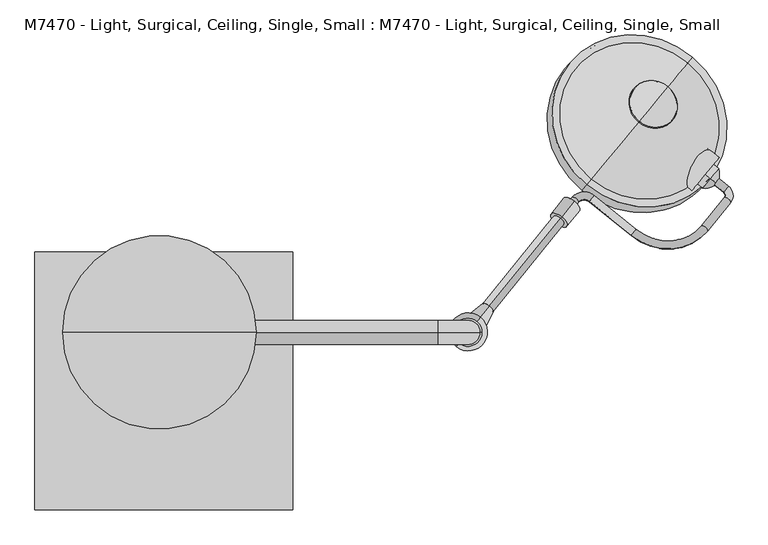
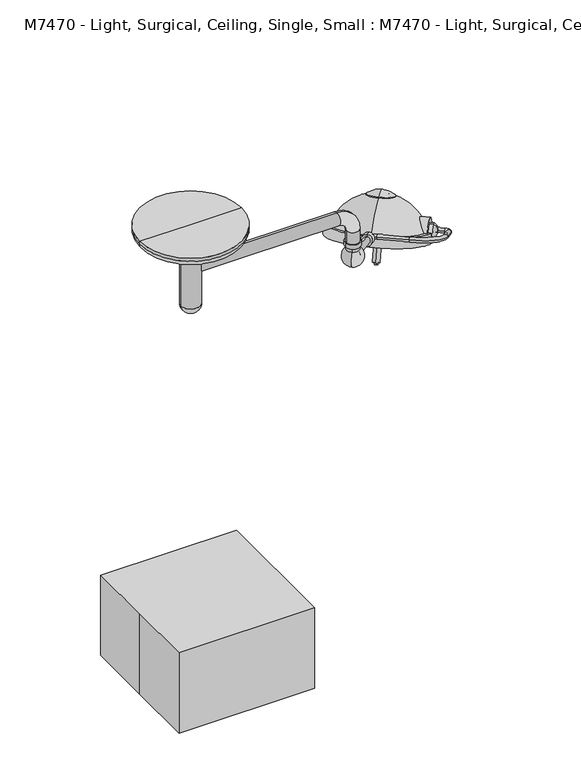
"""IFC4 building model written with IfcOpenShell, lengths in millimetres: proxy geometry, M7470 - Light, Surgical, Ceiling, Single, Small : M7470 - Light, Surgical, Ceiling, Single, Small."""

from ifc_helpers import new_model, si_unit, point, frame, frame_2d, origin, origin_with_axes, origin_2d, place, context, project, spatial, polyline, circle_curve, ellipse_curve, trimmed, segment, composite_curve, outline, extrude, source, transform, mapped, element, save
from ifc_brep_helpers import plane_surface, cylinder_surface, revolved_surface, advanced_brep


def m7470_light_surgical_ceiling_single_small_m7470_light_7ae27e33(model_context):
    return source(origin(), model_context, "Body", "SolidModel", [
        advanced_brep(
        [(1740.835031, 642.2802758, 1801.3604265), (1726.2322463, 624.2473385, 1811.6915373), (1762.8864892, 594.5653179, 1811.6915373), (1777.4892739, 612.5982552, 1801.3604265), (1765.4548505, 577.5564802, 1816.8570926), (1785.194358, 561.5717423, 1816.8570926), (1692.9754347, 488.0518556, 1868.1344952), (1712.7149421, 472.0671177, 1868.1344952), (1486.9216817, 475.7626592, 1930.1211596), (1472.318897, 457.7297218, 1940.4522704), (1355.271585, 582.3708055, 1930.1211596), (1340.6688003, 564.3378681, 1940.4522704), (1286.5870007, 578.2744067, 1950.7833811), (1306.3265081, 562.2896687, 1950.7833811), (1251.0372497, 494.0131207, 1989.8991704), (1231.2977423, 509.9978587, 1989.8991704)],
        [
            (0, 1, circle_curve(frame((1733.5336387, 633.2638072, 1806.5259819), z_axis=(-0.7771459614569792, 0.6293203910498273, 0.0), x_axis=(-0.5749127846454345, -0.7099581630143155, 0.40673664307580054)), 12.7)),
            (1, 0, circle_curve(frame((1733.5336387, 633.2638072, 1806.5259819), z_axis=(-0.7771459614569792, 0.6293203910498273, 0.0), x_axis=(-0.5749127846454345, -0.7099581630143155, 0.40673664307580054)), 12.7)),
            (1, 2),
            (2, 3, circle_curve(frame((1770.1878816, 603.5817865, 1806.5259819), z_axis=(-0.7771459614569792, 0.6293203910498273, 0.0), x_axis=(-0.5749127846454345, -0.7099581630143155, 0.40673664307580054)), 12.7)),
            (3, 0),
            (3, 2, circle_curve(frame((1770.1878816, 603.5817865, 1806.5259819), z_axis=(-0.7771459614569792, 0.6293203910498273, 0.0), x_axis=(-0.5749127846454345, -0.7099581630143155, 0.40673664307580054)), 12.7)),
            (4, 5, circle_curve(frame((1775.3246043, 569.5641113, 1816.8570926), z_axis=(0.574912784645419, 0.709958163014328, -0.4067366430758005), x_axis=(-0.7771459614569908, 0.6293203910498131, 0.0)), 12.7)),
            (5, 3, circle_curve(frame((1755.5850968, 585.5488492, 1816.8570926), z_axis=(0.2559676632747577, 0.31609373954292624, 0.9135454576426008), x_axis=(0.5749127846454357, 0.7099581630143145, -0.4067366430758004)), 38.1)),
            (2, 4, circle_curve(frame((1755.5850968, 585.5488492, 1816.8570926), z_axis=(-0.2559676632747577, -0.31609373954292624, -0.9135454576426008), x_axis=(0.5749127846454357, 0.7099581630143145, -0.4067366430758004)), 12.7)),
            (5, 4, circle_curve(frame((1775.3246043, 569.5641113, 1816.8570926), z_axis=(0.5749127846454273, 0.7099581630143212, -0.4067366430758005), x_axis=(-0.7771459614569847, 0.6293203910498207, 0.0)), 12.7)),
            (4, 6),
            (6, 7, circle_curve(frame((1702.8451884, 480.0594867, 1868.1344952), z_axis=(0.5749127846454346, 0.7099581630143152, -0.40673664307580043), x_axis=(-0.777145961456979, 0.6293203910498273, 0.0)), 12.7)),
            (7, 5),
            (7, 6, circle_curve(frame((1702.8451884, 480.0594867, 1868.1344952), z_axis=(0.5749127846454346, 0.7099581630143152, -0.40673664307580043), x_axis=(-0.777145961456979, 0.6293203910498273, 0.0)), 12.7)),
            (8, 9, circle_curve(frame((1479.6202894, 466.7461905, 1935.286715), z_axis=(0.7771459614569775, -0.6293203910498295, 0.0), x_axis=(0.5749127846454369, 0.7099581630143138, -0.4067366430758004)), 12.7)),
            (9, 7, circle_curve(frame((1574.5383901, 583.9602832, 1868.1344952), z_axis=(0.2559676632747577, 0.31609373954292624, 0.9135454576426008), x_axis=(0.7771459614569818, -0.6293203910498242, 0.0)), 177.8)),
            (6, 8, circle_curve(frame((1574.5383901, 583.9602832, 1868.1344952), z_axis=(-0.2559676632747577, -0.31609373954292624, -0.9135454576426008), x_axis=(0.7771459614569818, -0.6293203910498242, 0.0)), 152.4)),
            (9, 8, circle_curve(frame((1479.6202894, 466.7461905, 1935.286715), z_axis=(0.7771459614569785, -0.6293203910498282, 0.0), x_axis=(0.5749127846454356, 0.7099581630143149, -0.4067366430758004)), 12.7)),
            (8, 10),
            (10, 11, circle_curve(frame((1347.9701926, 573.3543368, 1935.286715), z_axis=(0.777145961456978, -0.6293203910498286, 0.0), x_axis=(0.574912784645436, 0.7099581630143144, -0.4067366430758003)), 12.7)),
            (11, 9),
            (11, 10, circle_curve(frame((1347.9701926, 573.3543368, 1935.286715), z_axis=(0.777145961456978, -0.6293203910498286, 0.0), x_axis=(0.574912784645436, 0.7099581630143144, -0.4067366430758003)), 12.7)),
            (12, 13, circle_curve(frame((1296.4567544, 570.2820377, 1950.7833811), z_axis=(0.5749127846454385, 0.7099581630143121, -0.40673664307580054), x_axis=(-0.7771459614569765, 0.629320391049831, 0.0)), 12.7)),
            (13, 11, circle_curve(frame((1326.0660155, 546.3049308, 1950.7833811), z_axis=(-0.2559676632747577, -0.31609373954292624, -0.9135454576426008), x_axis=(0.5749127846454407, 0.7099581630143105, -0.4067366430758004)), 25.4)),
            (10, 12, circle_curve(frame((1326.0660155, 546.3049308, 1950.7833811), z_axis=(0.2559676632747577, 0.31609373954292624, 0.9135454576426008), x_axis=(0.5749127846454407, 0.7099581630143105, -0.4067366430758004)), 50.8)),
            (13, 12, circle_curve(frame((1296.4567544, 570.2820377, 1950.7833811), z_axis=(0.5749127846454364, 0.7099581630143139, -0.40673664307580054), x_axis=(-0.777145961456978, 0.6293203910498291, 0.0)), 12.7)),
            (14, 15, circle_curve(frame((1241.167496, 502.0054897, 1989.8991704), z_axis=(-0.5749127846454374, -0.7099581630143132, 0.40673664307580004), x_axis=(-0.7771459614569771, 0.6293203910498298, 0.0)), 12.7)),
            (15, 14, circle_curve(frame((1241.167496, 502.0054897, 1989.8991704), z_axis=(-0.5749127846454374, -0.7099581630143132, 0.40673664307580004), x_axis=(-0.7771459614569771, 0.6293203910498298, 0.0)), 12.7)),
            (12, 15),
            (14, 13),
        ],
        [
            plane_surface(frame((1306.7585861, 106.2405083, 283.3710423), z_axis=(-0.7771459614569792, 0.6293203910498271, 0.0), x_axis=(0.2559676632747578, 0.3160937395429264, 0.9135454576426008))),
            cylinder_surface(frame((1733.5336387, 633.2638072, 1806.5259819), z_axis=(-0.7771459614569792, 0.6293203910498273, 0.0), x_axis=(-0.5749127846454345, -0.7099581630143155, 0.40673664307580054)), 12.7),
            revolved_surface(trimmed(ellipse_curve(frame((1770.1878816, 603.5817865, 1806.5259819), z_axis=(0.7771459614569786, -0.6293203910498283, 0.0), x_axis=(-0.5749127846454356, -0.7099581630143146, 0.40673664307580043)), 12.7, 12.7), [point((1777.4892739, 612.5982552, 1801.3604265))], [point((1762.8864892, 594.5653179, 1811.6915373))], True, "CARTESIAN"), (1328.8100443, 58.5255503, 293.7021531), (0.25596766327475773, 0.3160937395429263, 0.913545457642601)),
            revolved_surface(trimmed(ellipse_curve(frame((1770.1878816, 603.5817865, 1806.5259819), z_axis=(0.7771459614569786, -0.6293203910498283, 0.0), x_axis=(-0.5749127846454356, -0.7099581630143146, 0.40673664307580043)), 12.7, 12.7), [point((1762.8864892, 594.5653179, 1811.6915373))], [point((1777.4892739, 612.5982552, 1801.3604265))], True, "CARTESIAN"), (1328.8100443, 58.5255503, 293.7021531), (0.25596766327475773, 0.3160937395429263, 0.913545457642601)),
            cylinder_surface(frame((1775.3246043, 569.5641113, 1816.8570926), z_axis=(0.5749127846454346, 0.7099581630143152, -0.40673664307580043), x_axis=(-0.777145961456979, 0.6293203910498273, 0.0)), 12.7),
            revolved_surface(trimmed(ellipse_curve(frame((1702.8451884, 480.0594867, 1868.1344952), z_axis=(-0.5749127846454308, -0.7099581630143185, 0.4067366430758007), x_axis=(-0.777145961456982, 0.6293203910498238, 0.0)), 12.7, 12.7), [point((1712.7149421, 472.0671177, 1868.1344952))], [point((1692.9754347, 488.0518556, 1868.1344952))], True, "CARTESIAN"), (1147.7633376, 56.9369844, 344.9795556), (0.25596766327475773, 0.3160937395429263, 0.913545457642601)),
            revolved_surface(trimmed(ellipse_curve(frame((1702.8451884, 480.0594867, 1868.1344952), z_axis=(-0.5749127846454308, -0.7099581630143185, 0.4067366430758007), x_axis=(-0.777145961456982, 0.6293203910498238, 0.0)), 12.7, 12.7), [point((1692.9754347, 488.0518556, 1868.1344952))], [point((1712.7149421, 472.0671177, 1868.1344952))], True, "CARTESIAN"), (1147.7633376, 56.9369844, 344.9795556), (0.25596766327475773, 0.3160937395429263, 0.913545457642601)),
            cylinder_surface(frame((1479.6202894, 466.7461905, 1935.286715), z_axis=(0.7771459614569782, -0.6293203910498287, 0.0), x_axis=(0.574912784645436, 0.7099581630143144, -0.4067366430758003)), 12.7),
            revolved_surface(trimmed(ellipse_curve(frame((1347.9701926, 573.3543368, 1935.286715), z_axis=(-0.777145961456975, 0.629320391049833, 0.0), x_axis=(0.5749127846454405, 0.7099581630143107, -0.4067366430758002)), 12.7, 12.7), [point((1340.6688003, 564.3378681, 1940.4522704))], [point((1355.271585, 582.3708055, 1930.1211596))], True, "CARTESIAN"), (899.290963, 19.2816319, 427.6284415), (-0.25596766327475773, -0.3160937395429263, -0.913545457642601)),
            revolved_surface(trimmed(ellipse_curve(frame((1347.9701926, 573.3543368, 1935.286715), z_axis=(-0.777145961456975, 0.629320391049833, 0.0), x_axis=(0.5749127846454405, 0.7099581630143107, -0.4067366430758002)), 12.7, 12.7), [point((1355.271585, 582.3708055, 1930.1211596))], [point((1340.6688003, 564.3378681, 1940.4522704))], True, "CARTESIAN"), (899.290963, 19.2816319, 427.6284415), (-0.25596766327475773, -0.3160937395429263, -0.913545457642601)),
            plane_surface(frame((814.3924435, -25.0178092, 466.7442308), z_axis=(-0.5749127846454377, -0.7099581630143132, 0.4067366430758001), x_axis=(0.25596766327475756, 0.3160937395429259, 0.9135454576426011))),
            cylinder_surface(frame((1296.4567544, 570.2820377, 1950.7833811), z_axis=(0.5749127846454374, 0.7099581630143132, -0.40673664307580004), x_axis=(-0.7771459614569771, 0.6293203910498298, 0.0)), 12.7),
        ],
        [
            (0, [[1, 2]]),
            (1, [[3, 4, 5, -2]]),
            (1, [[-5, 6, -3, -1]]),
            (2, [[7, 8, -4, 9]]),
            (3, [[10, -9, -6, -8]]),
            (4, [[11, 12, 13, -7]]),
            (4, [[-13, 14, -11, -10]]),
            (5, [[15, 16, -12, 17]]),
            (6, [[18, -17, -14, -16]]),
            (7, [[19, 20, 21, -15]]),
            (7, [[-21, 22, -19, -18]]),
            (8, [[23, 24, -20, 25]]),
            (9, [[26, -25, -22, -24]]),
            (10, [[27, 28]]),
            (11, [[29, -27, 30, -23]]),
            (11, [[-30, -28, -29, -26]]),
        ],
    ),
        advanced_brep(
        [(1721.261074, 637.7345795, 1763.693259), (1705.2225201, 651.0325107, 1763.693259), (1705.2225201, 651.0325107, 1844.9108067), (1721.261074, 637.7345795, 1844.9108067), (1741.0506282, 621.3266083, 1804.3020328), (1705.2225201, 651.0325107, 1804.3020328)],
        [
            (0, 1),
            (1, 2, circle_curve(frame((1705.2225201, 651.0325107, 1804.3020328), z_axis=(0.7698129796821993, -0.6382695169854298, 0.0), x_axis=(0.0, 0.0, 1.0)), 40.6087738)),
            (2, 3),
            (3, 0, circle_curve(frame((1721.261074, 637.7345795, 1804.3020328), z_axis=(-0.7698129796821993, 0.6382695169854298, 0.0), x_axis=(0.0, 0.0, 1.0)), 40.6087738)),
            (2, 1, circle_curve(frame((1705.2225201, 651.0325107, 1804.3020328), z_axis=(0.7698129796821993, -0.6382695169854298, 0.0), x_axis=(0.0, 0.0, 1.0)), 40.6087738)),
            (0, 3, circle_curve(frame((1721.261074, 637.7345795, 1804.3020328), z_axis=(-0.7698129796821993, 0.6382695169854298, 0.0), x_axis=(0.0, 0.0, 1.0)), 40.6087738)),
            (4, 0, circle_curve(frame((1698.880381, 656.290923, 1810.5387051), z_axis=(0.6382695169854301, 0.769812979682199, 0.0), x_axis=(-0.7698129796821991, 0.63826951698543, 0.0)), 55.1337385)),
            (3, 4, circle_curve(frame((1698.880381, 656.290923, 1798.0653606), z_axis=(0.6382695169854297, 0.7698129796821994, 0.0), x_axis=(-0.7698129796821995, 0.6382695169854296, 0.0)), 55.1337385)),
            (1, 5),
            (5, 2),
        ],
        [
            cylinder_surface(frame((1705.2225201, 651.0325107, 1804.3020328), z_axis=(0.7698129796821993, -0.6382695169854298, 0.0), x_axis=(0.0, 0.0, 1.0)), 40.6087738),
            revolved_surface(trimmed(ellipse_curve(frame((1698.880381, 656.290923, 1798.0653606), z_axis=(0.6382695169854297, 0.7698129796821994, 0.0), x_axis=(-0.7698129796821995, 0.6382695169854296, 0.0)), 55.1337385, 55.1337385), [point((1721.261074, 637.7345795, 1844.9108067))], [point((1741.0506282, 621.3266083, 1804.3020328))], True, "CARTESIAN"), (1705.2225201, 651.0325107, 1804.3020328), (0.7698129796821993, -0.6382695169854298, 0.0)),
            revolved_surface(trimmed(ellipse_curve(frame((1698.880381, 656.290923, 1798.0653606), z_axis=(0.6382695169854296, 0.7698129796821995, 0.0), x_axis=(-0.7698129796821996, 0.6382695169854294, 0.0)), 55.1337385, 55.1337385), [point((1721.261074, 637.7345795, 1844.9108067))], [point((1741.0506282, 621.3266083, 1804.3020328))], True, "CARTESIAN"), (1705.2225201, 651.0325107, 1804.3020328), (0.7698129796821993, -0.6382695169854298, 0.0)),
            plane_surface(frame((1705.2225201, 651.0325107, 1804.3020328), z_axis=(-0.7698129796821992, 0.6382695169854299, 0.0), x_axis=(0.0, 0.0, 1.0))),
        ],
        [
            (0, [[1, 2, 3, 4]]),
            (0, [[-3, 5, -1, 6]]),
            (1, [[7, -4, 8]]),
            (2, [[-8, -6, -7]]),
            (3, [[9, 10, -2]]),
            (3, [[-10, -9, -5]]),
        ],
    ),
        advanced_brep(
        [(1496.9081674, 817.6344001, 1984.2946884), (1549.4769053, 881.037235, 1978.868084), (1587.2262401, 926.5664779, 1921.2927814), (1495.0601272, 815.4054901, 1981.6876662), (1587.2262401, 926.5664779, 1917.3966478), (1545.2418093, 875.9293114, 1963.9650044)],
        [
            (0, 1, circle_curve(frame((1514.8788649, 839.308749, 1783.8916913), z_axis=(-0.7698129796821976, 0.6382695169854321, 0.0), x_axis=(0.42708566892083927, 0.5151054258776686, -0.7431448254773932)), 202.3711557)),
            (1, 2, circle_curve(frame((1480.1450063, 797.4164536, 1808.1205002), z_axis=(-0.7698129796821995, 0.6382695169854299, 0.0), x_axis=(-0.6382695169854299, -0.7698129796821994, 0.0)), 202.3711557)),
            (2, 0, circle_curve(frame((1542.0672038, 872.100439, 1952.7937349), z_axis=(0.25960760071626565, 0.31311114715211635, 0.9135454576426013), x_axis=(0.5830882179937766, 0.7032591508229892, -0.4067366430757995)), 77.4480344)),
            (0, 2, circle_curve(frame((1542.0672038, 872.100439, 1952.7937349), z_axis=(0.25960760071626565, 0.31311114715211635, 0.9135454576426013), x_axis=(0.5830882179937766, 0.7032591508229892, -0.4067366430757995)), 77.4480344)),
            (3, 0),
            (2, 4),
            (4, 3, circle_curve(frame((1541.1431837, 870.985984, 1949.542157), z_axis=(0.25960760071626565, 0.31311114715211635, 0.9135454576426013), x_axis=(0.5830882179937766, 0.7032591508229892, -0.4067366430757995)), 79.0327347)),
            (3, 4, circle_curve(frame((1541.1431837, 870.985984, 1949.542157), z_axis=(0.25960760071626565, 0.31311114715211635, 0.9135454576426013), x_axis=(0.5830882179937766, 0.7032591508229892, -0.4067366430757995)), 79.0327347)),
            (5, 3, circle_curve(frame((1480.6908648, 798.0748102, 1698.5639329), z_axis=(0.7698129796821976, -0.6382695169854321, 0.0), x_axis=(0.42708566892083927, 0.5151054258776686, -0.7431448254773932)), 284.0173877)),
            (4, 5, circle_curve(frame((1462.5480105, 776.192824, 1711.2195886), z_axis=(0.7698129796821995, -0.6382695169854299, 0.0), x_axis=(-0.6382695169854299, -0.7698129796821994, 0.0)), 284.0173877)),
        ],
        [
            revolved_surface(trimmed(ellipse_curve(frame((1480.1450063, 797.4164536, 1808.1205002), z_axis=(-0.7698129796821995, 0.6382695169854299, 0.0), x_axis=(-0.6382695169854299, -0.7698129796821994, 0.0)), 202.3711557, 202.3711557), [point((1549.4769053, 881.037235, 1978.868084))], [point((1587.2262401, 926.5664779, 1921.2927814))], True, "CARTESIAN"), (1516.9910853, 841.8562852, 1864.5521965), (-0.25960760071626565, -0.31311114715211635, -0.9135454576426013)),
            revolved_surface(trimmed(ellipse_curve(frame((1480.1450063, 797.4164536, 1808.1205002), z_axis=(-0.7698129796821993, 0.6382695169854298, 0.0), x_axis=(-0.6382695169854298, -0.7698129796821993, 0.0)), 202.3711557, 202.3711557), [point((1549.4769053, 881.037235, 1978.868084))], [point((1587.2262401, 926.5664779, 1921.2927814))], True, "CARTESIAN"), (1516.9910853, 841.8562852, 1864.5521965), (-0.25960760071626565, -0.31311114715211635, -0.9135454576426013)),
            revolved_surface(polyline([(1587.2262401, 926.5664779, 1921.2927814), (1587.2262401, 926.5664779, 1917.3966478)]), (1516.9910853, 841.8562852, 1864.5521965), (-0.25960760071626565, -0.31311114715211635, -0.9135454576426013)),
            revolved_surface(trimmed(ellipse_curve(frame((1462.5480105, 776.192824, 1711.2195886), z_axis=(0.7698129796821995, -0.6382695169854299, 0.0), x_axis=(-0.6382695169854299, -0.7698129796821994, 0.0)), 284.0173877, 284.0173877), [point((1587.2262401, 926.5664779, 1917.3966478))], [point((1545.2418093, 875.9293114, 1963.9650044))], True, "CARTESIAN"), (1516.9910853, 841.8562852, 1864.5521965), (-0.25960760071626565, -0.31311114715211635, -0.9135454576426013)),
            revolved_surface(trimmed(ellipse_curve(frame((1462.5480105, 776.192824, 1711.2195886), z_axis=(0.7698129796821993, -0.6382695169854298, 0.0), x_axis=(-0.6382695169854298, -0.7698129796821993, 0.0)), 284.0173877, 284.0173877), [point((1587.2262401, 926.5664779, 1917.3966478))], [point((1545.2418093, 875.9293114, 1963.9650044))], True, "CARTESIAN"), (1516.9910853, 841.8562852, 1864.5521965), (-0.25960760071626565, -0.31311114715211635, -0.9135454576426013)),
        ],
        [
            (0, [[1, 2, 3]]),
            (1, [[-2, -1, 4]]),
            (2, [[5, -3, 6, 7]]),
            (2, [[-6, -4, -5, 8]]),
            (3, [[9, -7, 10]]),
            (4, [[-10, -8, -9]]),
        ],
    ),
        advanced_brep(
        [(1448.7501126, 759.5512633, 1624.4158117), (1456.1553329, 768.4826545, 1619.2502563), (1441.3448922, 750.6198721, 1629.5813671), (1451.1647669, 762.4635632, 1609.2425198), (1445.5510315, 755.6928711, 1613.1584142), (1439.9372961, 748.922179, 1617.0743086)],
        [
            (0, 1),
            (1, 2, circle_curve(frame((1448.7501126, 759.5512633, 1624.4158117), z_axis=(0.2596076007162656, 0.31311114715211635, 0.9135454576426013), x_axis=(-0.5830882179937766, -0.7032591508229892, 0.40673664307579943)), 12.7)),
            (2, 0),
            (2, 1, circle_curve(frame((1448.7501126, 759.5512633, 1624.4158117), z_axis=(0.2596076007162656, 0.31311114715211635, 0.9135454576426013), x_axis=(-0.5830882179937766, -0.7032591508229892, 0.40673664307579943)), 12.7)),
            (3, 4),
            (4, 5),
            (5, 3, circle_curve(frame((1445.5510315, 755.6928711, 1613.1584142), z_axis=(-0.2596076007162656, -0.31311114715211635, -0.9135454576426013), x_axis=(-0.5830882179937766, -0.7032591508229892, 0.40673664307579943)), 9.6275919)),
            (3, 5, circle_curve(frame((1445.5510315, 755.6928711, 1613.1584142), z_axis=(-0.2596076007162656, -0.31311114715211635, -0.9135454576426013), x_axis=(-0.5830882179937766, -0.7032591508229892, 0.40673664307579943)), 9.6275919)),
            (1, 3),
            (5, 2),
        ],
        [
            plane_surface(frame((1448.7501126, 759.5512633, 1624.4158117), z_axis=(0.25960760071626565, 0.31311114715211635, 0.9135454576426012), x_axis=(-0.5830882179937766, -0.7032591508229892, 0.40673664307579943))),
            plane_surface(frame((1445.5510315, 755.6928711, 1613.1584142), z_axis=(-0.25960760071626565, -0.31311114715211635, -0.9135454576426012), x_axis=(-0.5830882179937766, -0.7032591508229892, 0.40673664307579943))),
            revolved_surface(polyline([(1439.9372961, 748.922179, 1617.0743086), (1441.3448922, 750.6198721, 1629.5813671)]), (1475.1262448, 791.3633558, 1717.2320302), (0.2596076007162656, 0.31311114715211635, 0.9135454576426013)),
        ],
        [
            (0, [[1, 2, 3]]),
            (0, [[-3, 4, -1]]),
            (1, [[5, 6, 7]]),
            (1, [[-6, -5, 8]]),
            (2, [[9, -7, 10, -2]]),
            (2, [[-10, -8, -9, -4]]),
        ],
    ),
        advanced_brep(
        [(1475.1262448, 791.3633558, 1717.2320302), (1486.2340754, 804.7604427, 1709.4836971), (1464.0184142, 777.966269, 1724.9803632), (1459.8579431, 772.9483501, 1616.6674786), (1448.7501126, 759.5512633, 1624.4158117), (1437.642282, 746.1541765, 1632.1641447)],
        [
            (0, 1),
            (1, 2, circle_curve(frame((1475.1262448, 791.3633558, 1717.2320302), z_axis=(0.2596076007162656, 0.31311114715211635, 0.9135454576426013), x_axis=(-0.5830882179937766, -0.7032591508229892, 0.40673664307579943)), 19.05)),
            (2, 0),
            (2, 1, circle_curve(frame((1475.1262448, 791.3633558, 1717.2320302), z_axis=(0.2596076007162656, 0.31311114715211635, 0.9135454576426013), x_axis=(-0.5830882179937766, -0.7032591508229892, 0.40673664307579943)), 19.05)),
            (3, 4),
            (4, 5),
            (5, 3, circle_curve(frame((1448.7501126, 759.5512633, 1624.4158117), z_axis=(-0.2596076007162656, -0.31311114715211635, -0.9135454576426013), x_axis=(-0.5830882179937766, -0.7032591508229892, 0.40673664307579943)), 19.05)),
            (3, 5, circle_curve(frame((1448.7501126, 759.5512633, 1624.4158117), z_axis=(-0.2596076007162656, -0.31311114715211635, -0.9135454576426013), x_axis=(-0.5830882179937766, -0.7032591508229892, 0.40673664307579943)), 19.05)),
            (1, 3),
            (5, 2),
        ],
        [
            plane_surface(frame((1475.1262448, 791.3633558, 1717.2320302), z_axis=(0.25960760071626565, 0.31311114715211635, 0.9135454576426012), x_axis=(-0.5830882179937766, -0.7032591508229892, 0.40673664307579943))),
            plane_surface(frame((1448.7501126, 759.5512633, 1624.4158117), z_axis=(-0.25960760071626565, -0.31311114715211635, -0.9135454576426012), x_axis=(-0.5830882179937766, -0.7032591508229892, 0.40673664307579943))),
            cylinder_surface(frame((1475.1262448, 791.3633558, 1717.2320302), z_axis=(0.2596076007162656, 0.31311114715211635, 0.9135454576426013), x_axis=(-0.5830882179937766, -0.7032591508229892, 0.40673664307579943)), 19.05),
        ],
        [
            (0, [[1, 2, 3]]),
            (0, [[-3, 4, -1]]),
            (1, [[5, 6, 7]]),
            (1, [[-6, -5, 8]]),
            (2, [[9, -7, 10, -2]]),
            (2, [[-10, -8, -9, -4]]),
        ],
    ),
        advanced_brep(
        [(1480.0717696, 797.3281232, 1734.6350712), (1505.9900409, 828.5879925, 1716.5556274), (1454.1534983, 766.0682539, 1752.7145149), (1501.0445161, 822.6232251, 1699.1525864), (1475.1262448, 791.3633558, 1717.2320302), (1449.2079735, 760.1034866, 1735.311474)],
        [
            (0, 1),
            (1, 2, circle_curve(frame((1480.0717696, 797.3281232, 1734.6350712), z_axis=(0.2596076007162652, 0.31311114715211585, 0.9135454576426016), x_axis=(-0.5830882179937769, -0.7032591508229895, 0.4067366430757988)), 44.45)),
            (2, 0),
            (2, 1, circle_curve(frame((1480.0717696, 797.3281232, 1734.6350712), z_axis=(0.2596076007162652, 0.31311114715211585, 0.9135454576426016), x_axis=(-0.5830882179937769, -0.7032591508229895, 0.4067366430757988)), 44.45)),
            (3, 4),
            (4, 5),
            (5, 3, circle_curve(frame((1475.1262448, 791.3633558, 1717.2320302), z_axis=(-0.2596076007162652, -0.31311114715211585, -0.9135454576426016), x_axis=(-0.5830882179937769, -0.7032591508229895, 0.4067366430757988)), 44.45)),
            (3, 5, circle_curve(frame((1475.1262448, 791.3633558, 1717.2320302), z_axis=(-0.2596076007162652, -0.31311114715211585, -0.9135454576426016), x_axis=(-0.5830882179937769, -0.7032591508229895, 0.4067366430757988)), 44.45)),
            (1, 3),
            (5, 2),
        ],
        [
            plane_surface(frame((1480.0717696, 797.3281232, 1734.6350712), z_axis=(0.25960760071626526, 0.31311114715211585, 0.9135454576426016), x_axis=(-0.5830882179937769, -0.7032591508229895, 0.4067366430757988))),
            plane_surface(frame((1475.1262448, 791.3633558, 1717.2320302), z_axis=(-0.25960760071626526, -0.31311114715211585, -0.9135454576426016), x_axis=(-0.5830882179937769, -0.7032591508229895, 0.4067366430757988))),
            cylinder_surface(frame((1480.0717696, 797.3281232, 1734.6350712), z_axis=(0.2596076007162652, 0.31311114715211585, 0.9135454576426016), x_axis=(-0.5830882179937769, -0.7032591508229895, 0.4067366430757988)), 44.45),
        ],
        [
            (0, [[1, 2, 3]]),
            (0, [[-3, 4, -1]]),
            (1, [[5, 6, 7]]),
            (1, [[-6, -5, 8]]),
            (2, [[9, -7, 10, -2]]),
            (2, [[-10, -8, -9, -4]]),
        ],
    ),
        advanced_brep(
        [(1483.0837441, 800.9608473, 1745.2340505), (1516.4072357, 841.1521078, 1721.9890514), (1449.7602524, 760.7695868, 1768.4790497), (1510.3832868, 833.8866596, 1713.4910927), (1480.0717696, 797.3281232, 1734.6350712), (1449.7602524, 760.7695868, 1755.7790497)],
        [
            (0, 1),
            (1, 2, circle_curve(frame((1483.0837441, 800.9608473, 1745.2340505), z_axis=(0.25960760071626576, 0.3131111471521165, 0.9135454576426012), x_axis=(-0.5830882179937765, -0.7032591508229892, 0.40673664307579965)), 57.15)),
            (2, 0),
            (2, 1, circle_curve(frame((1483.0837441, 800.9608473, 1745.2340505), z_axis=(0.25960760071626576, 0.3131111471521165, 0.9135454576426012), x_axis=(-0.5830882179937765, -0.7032591508229892, 0.40673664307579965)), 57.15)),
            (3, 4),
            (4, 5),
            (5, 3, circle_curve(frame((1480.0717696, 797.3281232, 1734.6350712), z_axis=(-0.25960760071626576, -0.3131111471521165, -0.9135454576426012), x_axis=(-0.5830882179937765, -0.7032591508229892, 0.40673664307579965)), 51.9844446)),
            (3, 5, circle_curve(frame((1480.0717696, 797.3281232, 1734.6350712), z_axis=(-0.25960760071626576, -0.3131111471521165, -0.9135454576426012), x_axis=(-0.5830882179937765, -0.7032591508229892, 0.40673664307579965)), 51.9844446)),
            (1, 3),
            (5, 2),
        ],
        [
            plane_surface(frame((1483.0837441, 800.9608473, 1745.2340505), z_axis=(0.25960760071626576, 0.3131111471521165, 0.9135454576426012), x_axis=(-0.5830882179937765, -0.7032591508229892, 0.40673664307579965))),
            plane_surface(frame((1480.0717696, 797.3281232, 1734.6350712), z_axis=(-0.25960760071626576, -0.3131111471521165, -0.9135454576426012), x_axis=(-0.5830882179937765, -0.7032591508229892, 0.40673664307579965))),
            revolved_surface(polyline([(1449.7602524, 760.7695868, 1755.7790497), (1449.7602524, 760.7695868, 1768.4790497)]), (1483.0837441, 800.9608473, 1745.2340505), (0.25960760071626576, 0.3131111471521165, 0.9135454576426012)),
        ],
        [
            (0, [[1, 2, 3]]),
            (0, [[-3, 4, -1]]),
            (1, [[5, 6, 7]]),
            (1, [[-6, -5, 8]]),
            (2, [[9, -7, 10, -2]]),
            (2, [[-10, -8, -9, -4]]),
        ],
    ),
        extrude(outline(composite_curve([segment(polyline([(25.1937137, 4.6953206), (-31.6273953, 132.317621)]), True, "CONTINUOUS"), segment(trimmed(circle_curve(frame_2d((0.0, 69.9387006)), 69.9387006), [point((-31.6273953, 132.317621))], [point((25.1937137, 4.6953206))], False, "CARTESIAN"), True, "CONTINUOUS")], self_intersect=False)), frame((1659.5038481, 595.8914987, 1800.6600142), z_axis=(-0.7698129796821992, 0.6382695169854299, 0.0), x_axis=(0.0, 0.0, 1.0)), (0.0, 0.0, 1.0), 84.2600986),
        advanced_brep(
        [(1346.1133009, 635.7616294, 1903.3370584), (1545.2465329, 875.9350086, 1963.9816266), (1649.727336, 1001.9486693, 1691.5492884), (1350.1582608, 640.640231, 1900.5154726), (1645.6823761, 997.0700677, 1694.3708742), (1543.5949178, 873.9430057, 1958.1696802)],
        [
            (0, 1, circle_curve(frame((1477.2351085, 793.9068435, 1679.3194701), z_axis=(-0.7698129796821976, 0.6382695169854323, 0.0), x_axis=(0.4270856689208392, 0.5151054258776685, -0.7431448254773935)), 303.9518334)),
            (1, 2, circle_curve(frame((1455.7322005, 767.972317, 1694.318951), z_axis=(-0.7698129796821995, 0.6382695169854298, 0.0), x_axis=(-0.6382695169854299, -0.7698129796821995, 0.0)), 303.9518334)),
            (2, 0, circle_curve(frame((1497.9203184, 818.8551493, 1797.4431734), z_axis=(0.2596076007162657, 0.31311114715211646, 0.9135454576426013), x_axis=(0.5830882179937766, 0.7032591508229892, -0.4067366430757996)), 260.35)),
            (0, 2, circle_curve(frame((1497.9203184, 818.8551493, 1797.4431734), z_axis=(0.2596076007162657, 0.31311114715211646, 0.9135454576426013), x_axis=(0.5830882179937766, 0.7032591508229892, -0.4067366430757996)), 260.35)),
            (3, 0),
            (2, 4),
            (4, 3, circle_curve(frame((1497.9203184, 818.8551493, 1797.4431734), z_axis=(0.2596076007162657, 0.31311114715211646, 0.9135454576426013), x_axis=(0.5830882179937766, 0.7032591508229892, -0.4067366430757996)), 253.412868)),
            (3, 4, circle_curve(frame((1497.9203184, 818.8551493, 1797.4431734), z_axis=(0.2596076007162657, 0.31311114715211646, 0.9135454576426013), x_axis=(0.5830882179937766, 0.7032591508229892, -0.4067366430757996)), 253.412868)),
            (5, 3, circle_curve(frame((1477.2351085, 793.9068435, 1679.3194701), z_axis=(0.7698129796821976, -0.6382695169854323, 0.0), x_axis=(0.4270856689208392, 0.5151054258776685, -0.7431448254773935)), 297.6018334)),
            (4, 5, circle_curve(frame((1455.7322005, 767.972317, 1694.318951), z_axis=(0.7698129796821995, -0.6382695169854298, 0.0), x_axis=(-0.6382695169854299, -0.7698129796821995, 0.0)), 297.6018334)),
        ],
        [
            revolved_surface(trimmed(ellipse_curve(frame((1455.7322005, 767.972317, 1694.318951), z_axis=(-0.7698129796821995, 0.6382695169854298, 0.0), x_axis=(-0.6382695169854299, -0.7698129796821995, 0.0)), 303.9518334, 303.9518334), [point((1545.2465329, 875.9350086, 1963.9816266))], [point((1649.727336, 1001.9486693, 1691.5492884))], True, "CARTESIAN"), (1497.9203184, 818.8551493, 1797.4431734), (-0.2596076007162657, -0.31311114715211646, -0.9135454576426013)),
            revolved_surface(trimmed(ellipse_curve(frame((1455.7322005, 767.972317, 1694.318951), z_axis=(-0.7698129796821995, 0.6382695169854299, 0.0), x_axis=(-0.6382695169854299, -0.7698129796821995, 0.0)), 303.9518334, 303.9518334), [point((1545.2465329, 875.9350086, 1963.9816266))], [point((1649.727336, 1001.9486693, 1691.5492884))], True, "CARTESIAN"), (1497.9203184, 818.8551493, 1797.4431734), (-0.2596076007162657, -0.31311114715211646, -0.9135454576426013)),
            plane_surface(frame((1497.9203184, 818.8551493, 1797.4431734), z_axis=(-0.25960760071626576, -0.31311114715211646, -0.9135454576426012), x_axis=(0.5830882179937766, 0.7032591508229892, -0.4067366430757996))),
            revolved_surface(trimmed(ellipse_curve(frame((1455.7322005, 767.972317, 1694.318951), z_axis=(0.7698129796821995, -0.6382695169854298, 0.0), x_axis=(-0.6382695169854299, -0.7698129796821995, 0.0)), 297.6018334, 297.6018334), [point((1645.6823761, 997.0700677, 1694.3708742))], [point((1543.5949178, 873.9430057, 1958.1696802))], True, "CARTESIAN"), (1497.9203184, 818.8551493, 1797.4431734), (-0.2596076007162657, -0.31311114715211646, -0.9135454576426013)),
            revolved_surface(trimmed(ellipse_curve(frame((1455.7322005, 767.972317, 1694.318951), z_axis=(0.7698129796821995, -0.6382695169854299, 0.0), x_axis=(-0.6382695169854299, -0.7698129796821995, 0.0)), 297.6018334, 297.6018334), [point((1645.6823761, 997.0700677, 1694.3708742))], [point((1543.5949178, 873.9430057, 1958.1696802))], True, "CARTESIAN"), (1497.9203184, 818.8551493, 1797.4431734), (-0.2596076007162657, -0.31311114715211646, -0.9135454576426013)),
        ],
        [
            (0, [[1, 2, 3]]),
            (1, [[-2, -1, 4]]),
            (2, [[5, -3, 6, 7]]),
            (2, [[-6, -4, -5, 8]]),
            (3, [[9, -7, 10]]),
            (4, [[-10, -8, -9]]),
        ],
    ),
        advanced_brep(
        [(1316.4662858, 600.0045449, 1861.4590463), (1331.3028602, 617.898847, 1913.6681692), (1664.5377767, 1019.8114517, 1681.2181777), (1649.7012024, 1001.9171496, 1629.0090547), (1320.168896, 604.4702405, 1858.8762686), (1645.9985922, 997.451454, 1631.5918324), (1333.3569621, 620.3762868, 1905.2843778), (1659.1866583, 1013.3575003, 1677.9999417), (1496.2718102, 816.8668936, 1791.6421598), (1497.9203184, 818.8551493, 1797.4431734)],
        [
            (0, 1),
            (1, 2, circle_curve(frame((1497.9203184, 818.8551493, 1797.4431734), z_axis=(-0.2596076007162655, -0.3131111471521162, -0.9135454576426014), x_axis=(0.5830882179937767, 0.7032591508229893, -0.4067366430757992)), 285.75)),
            (2, 3),
            (3, 0, circle_curve(frame((1483.0837441, 800.9608473, 1745.2340505), z_axis=(0.2596076007162655, 0.3131111471521162, 0.9135454576426014), x_axis=(0.5830882179937767, 0.7032591508229893, -0.4067366430757992)), 285.75)),
            (2, 1, circle_curve(frame((1497.9203184, 818.8551493, 1797.4431734), z_axis=(-0.2596076007162655, -0.3131111471521162, -0.9135454576426014), x_axis=(0.5830882179937767, 0.7032591508229893, -0.4067366430757992)), 285.75)),
            (0, 3, circle_curve(frame((1483.0837441, 800.9608473, 1745.2340505), z_axis=(0.2596076007162655, 0.3131111471521162, 0.9135454576426014), x_axis=(0.5830882179937767, 0.7032591508229893, -0.4067366430757992)), 285.75)),
            (4, 0),
            (3, 5),
            (5, 4, circle_curve(frame((1483.0837441, 800.9608473, 1745.2340505), z_axis=(0.2596076007162655, 0.3131111471521162, 0.9135454576426014), x_axis=(0.5830882179937767, 0.7032591508229893, -0.4067366430757992)), 279.4)),
            (4, 5, circle_curve(frame((1483.0837441, 800.9608473, 1745.2340505), z_axis=(0.2596076007162655, 0.3131111471521162, 0.9135454576426014), x_axis=(0.5830882179937767, 0.7032591508229893, -0.4067366430757992)), 279.4)),
            (6, 4),
            (5, 7),
            (7, 6, circle_curve(frame((1496.2718102, 816.8668936, 1791.6421598), z_axis=(0.2596076007162655, 0.3131111471521162, 0.9135454576426014), x_axis=(0.5830882179937767, 0.7032591508229893, -0.4067366430757992)), 279.4)),
            (6, 7, circle_curve(frame((1496.2718102, 816.8668936, 1791.6421598), z_axis=(0.2596076007162655, 0.3131111471521162, 0.9135454576426014), x_axis=(0.5830882179937767, 0.7032591508229893, -0.4067366430757992)), 279.4)),
            (8, 6),
            (7, 8),
            (1, 9),
            (9, 2),
        ],
        [
            cylinder_surface(frame((1483.0837441, 800.9608473, 1745.2340505), z_axis=(-0.2596076007162655, -0.3131111471521162, -0.9135454576426014), x_axis=(0.5830882179937767, 0.7032591508229893, -0.4067366430757992)), 285.75),
            plane_surface(frame((1483.0837441, 800.9608473, 1745.2340505), z_axis=(-0.2596076007162655, -0.3131111471521162, -0.9135454576426014), x_axis=(0.5830882179937767, 0.7032591508229893, -0.4067366430757992))),
            revolved_surface(polyline([(1645.9985921978723, 997.451454028378, 1631.5918323908784), (1659.1866583370233, 1013.3575003311619, 1677.9999417192307)]), (1483.0837441, 800.9608473, 1745.2340505), (-0.2596076007162655, -0.3131111471521162, -0.9135454576426014)),
            plane_surface(frame((1496.2718102, 816.8668936, 1791.6421598), z_axis=(-0.2596076007162655, -0.3131111471521162, -0.9135454576426014), x_axis=(0.5830882179937767, 0.7032591508229893, -0.4067366430757992))),
            plane_surface(frame((1497.9203184, 818.8551493, 1797.4431734), z_axis=(0.2596076007162655, 0.3131111471521162, 0.9135454576426014), x_axis=(0.5830882179937767, 0.7032591508229893, -0.4067366430757992))),
        ],
        [
            (0, [[1, 2, 3, 4]]),
            (0, [[-3, 5, -1, 6]]),
            (1, [[7, -4, 8, 9]]),
            (1, [[-8, -6, -7, 10]]),
            (2, [[11, -9, 12, 13]]),
            (2, [[-12, -10, -11, 14]]),
            (3, [[15, -13, 16]]),
            (3, [[-16, -14, -15]]),
            (4, [[17, 18, -2]]),
            (4, [[-18, -17, -5]]),
        ],
    ),
        advanced_brep(
        [(1235.7366669, 495.2989743, 1958.9919398), (1244.1809696, 505.7268197, 1987.767212), (1252.6252723, 516.1546651, 2016.5424843), (1275.5761712, 544.4966648, 1929.4720542), (1292.4647766, 565.3523556, 1987.0225987), (1284.0204739, 554.9245102, 1958.2473264)],
        [
            (0, 1),
            (1, 2),
            (2, 0, circle_curve(frame((1244.1809696, 505.7268197, 1987.767212), z_axis=(-0.5703579709494108, -0.7043334365325427, 0.42261826174069883), x_axis=(0.265962289743456, 0.32843607534975183, 0.9063077870366504)), 31.75)),
            (0, 2, circle_curve(frame((1244.1809696, 505.7268197, 1987.767212), z_axis=(-0.5703579709494108, -0.7043334365325427, 0.42261826174069883), x_axis=(0.265962289743456, 0.32843607534975183, 0.9063077870366504)), 31.75)),
            (3, 0),
            (2, 4),
            (4, 3, circle_curve(frame((1284.0204739, 554.9245102, 1958.2473264), z_axis=(-0.5703579709494108, -0.7043334365325427, 0.42261826174069883), x_axis=(0.265962289743456, 0.32843607534975183, 0.9063077870366504)), 31.75)),
            (3, 4, circle_curve(frame((1284.0204739, 554.9245102, 1958.2473264), z_axis=(-0.5703579709494108, -0.7043334365325427, 0.42261826174069883), x_axis=(0.265962289743456, 0.32843607534975183, 0.9063077870366504)), 31.75)),
            (5, 3),
            (4, 5),
        ],
        [
            plane_surface(frame((1244.1809696, 505.7268197, 1987.767212), z_axis=(-0.5703579709494109, -0.7043334365325429, 0.42261826174069894), x_axis=(0.265962289743456, 0.32843607534975183, 0.9063077870366504))),
            cylinder_surface(frame((1244.1809696, 505.7268197, 1987.767212), z_axis=(0.5703579709494108, 0.7043334365325427, -0.42261826174069883), x_axis=(0.265962289743456, 0.32843607534975183, 0.9063077870366504)), 31.75),
            plane_surface(frame((1284.0204739, 554.9245102, 1958.2473264), z_axis=(0.5703579709494109, 0.7043334365325429, -0.42261826174069894), x_axis=(0.265962289743456, 0.32843607534975183, 0.9063077870366504))),
        ],
        [
            (0, [[1, 2, 3]]),
            (0, [[-2, -1, 4]]),
            (1, [[5, -3, 6, 7]]),
            (1, [[-6, -4, -5, 8]]),
            (2, [[9, -7, 10]]),
            (2, [[-10, -8, -9]]),
        ],
    ),
        extrude(outline(composite_curve([segment(trimmed(circle_curve(origin_2d(), 20.2288163), [point((0.0, 20.2288163))], [point((0.0, -20.2288163))], False, "CARTESIAN"), True, "CONTINUOUS"), segment(trimmed(circle_curve(origin_2d(), 20.2288163), [point((0.0, -20.2288163))], [point((0.0, 20.2288163))], False, "CARTESIAN"), True, "CONTINUOUS")], self_intersect=False)), frame((1244.1809696, 505.7268197, 1987.767212), z_axis=(-0.5703579709494108, -0.7043334365325428, 0.4226182617406986), x_axis=(0.777145961456977, -0.62932039104983, 0.0)), (0.0, 0.0, 1.0), 393.7),
        advanced_brep(
        [(976.8515115, 175.602432, 2183.0066897), (985.8538291, 186.7193684, 2216.7067436), (967.849194, 164.4854957, 2149.3066358), (1024.9063629, 234.9452313, 2173.9001347), (1019.6310364, 228.4307457, 2154.1520217), (1014.35571, 221.9162601, 2134.4039086)],
        [
            (0, 1),
            (1, 2, circle_curve(frame((976.8515115, 175.602432, 2183.0066897), z_axis=(-0.5792924743379562, -0.7153666293621104, 0.3907311284892742), x_axis=(-0.24589506657621132, -0.3036551185209666, -0.9205048534524403)), 36.6104033)),
            (2, 0),
            (2, 1, circle_curve(frame((976.8515115, 175.602432, 2183.0066897), z_axis=(-0.5792924743379562, -0.7153666293621104, 0.3907311284892742), x_axis=(-0.24589506657621132, -0.3036551185209666, -0.9205048534524403)), 36.6104033)),
            (3, 4),
            (4, 5),
            (5, 3, circle_curve(frame((1019.6310364, 228.4307457, 2154.1520217), z_axis=(0.5792924743379562, 0.7153666293621104, -0.3907311284892742), x_axis=(-0.24589506657621132, -0.3036551185209666, -0.9205048534524403)), 21.4535676)),
            (3, 5, circle_curve(frame((1019.6310364, 228.4307457, 2154.1520217), z_axis=(0.5792924743379562, 0.7153666293621104, -0.3907311284892742), x_axis=(-0.24589506657621132, -0.3036551185209666, -0.9205048534524403)), 21.4535676)),
            (1, 3),
            (5, 2),
        ],
        [
            plane_surface(frame((976.8515115, 175.602432, 2183.0066897), z_axis=(-0.5792924743379563, -0.7153666293621104, 0.3907311284892742), x_axis=(-0.24589506657621132, -0.3036551185209666, -0.9205048534524403))),
            plane_surface(frame((1019.6310364, 228.4307457, 2154.1520217), z_axis=(0.5792924743379563, 0.7153666293621104, -0.3907311284892742), x_axis=(-0.24589506657621132, -0.3036551185209666, -0.9205048534524403))),
            revolved_surface(polyline([(1014.35571, 221.9162601, 2134.4039086), (967.849194, 164.4854957, 2149.3066358)]), (990.2029787, 192.0901209, 2174.001163), (-0.579292474337956, -0.7153666293621103, 0.3907311284892741)),
        ],
        [
            (0, [[1, 2, 3]]),
            (0, [[-3, 4, -1]]),
            (1, [[5, 6, 7]]),
            (1, [[-6, -5, 8]]),
            (2, [[9, -7, 10, -2]]),
            (2, [[-10, -8, -9, -4]]),
        ],
    ),
        advanced_brep(
        [(959.0523183, 153.6222589, 2277.562195), (983.0294252, 183.23152, 2277.562195), (935.0752114, 124.0129978, 2277.562195), (983.0294252, 183.23152, 2251.7869575), (959.0523183, 153.6222589, 2145.7286543), (935.0752114, 124.0129978, 2251.7869575)],
        [
            (0, 1),
            (1, 2, circle_curve(frame((959.0523183, 153.6222589, 2277.562195), z_axis=(0.0, 0.0, 1.0), x_axis=(-0.6293203910498301, -0.777145961456977, 0.0)), 38.1)),
            (2, 0),
            (2, 1, circle_curve(frame((959.0523183, 153.6222589, 2277.562195), z_axis=(0.0, 0.0, 1.0), x_axis=(-0.6293203910498301, -0.777145961456977, 0.0)), 38.1)),
            (3, 4, circle_curve(frame((959.0523183, 153.6222589, 2205.6012588), z_axis=(-0.7771459614569791, 0.6293203910498274, 0.0), x_axis=(0.6293203910498274, 0.7771459614569791, 0.0)), 59.8726045)),
            (4, 5, circle_curve(frame((959.0523183, 153.6222589, 2205.6012588), z_axis=(-0.7771459614569771, 0.62932039104983, 0.0), x_axis=(-0.62932039104983, -0.7771459614569771, 0.0)), 59.8726045)),
            (5, 3, circle_curve(frame((959.0523183, 153.6222589, 2251.7869575), z_axis=(0.0, 0.0, -1.0), x_axis=(-0.6293203910498301, -0.777145961456977, 0.0)), 38.1)),
            (3, 5, circle_curve(frame((959.0523183, 153.6222589, 2251.7869575), z_axis=(0.0, 0.0, -1.0), x_axis=(-0.6293203910498301, -0.777145961456977, 0.0)), 38.1)),
            (1, 3),
            (5, 2),
        ],
        [
            plane_surface(frame((959.0523183, 153.6222589, 2277.562195), z_axis=(0.0, 0.0, 1.0000000000000002), x_axis=(-0.6293203910498301, -0.777145961456977, 0.0))),
            revolved_surface(trimmed(ellipse_curve(frame((959.0523183, 153.6222589, 2205.6012588), z_axis=(-0.7771459614569771, 0.62932039104983, 0.0), x_axis=(-0.62932039104983, -0.7771459614569771, 0.0)), 59.8726045, 59.8726045), [point((959.0523183, 153.6222589, 2145.7286543))], [point((935.0752114, 124.0129978, 2251.7869575))], True, "CARTESIAN"), (959.0523183, 153.6222589, 2277.562195), (0.0, 0.0, 1.0)),
            cylinder_surface(frame((959.0523183, 153.6222589, 2277.562195), z_axis=(0.0, 0.0, 1.0), x_axis=(-0.6293203910498301, -0.777145961456977, 0.0)), 38.1),
        ],
        [
            (0, [[1, 2, 3]]),
            (0, [[-3, 4, -1]]),
            (1, [[5, 6, 7]]),
            (1, [[-6, -5, 8]]),
            (2, [[9, -7, 10, -2]]),
            (2, [[-10, -8, -9, -4]]),
        ],
    ),
        advanced_brep(
        [(912.6181725, 152.4, 2277.562195), (957.0681725, 152.4, 2277.562195), (1001.5181725, 152.4, 2277.562195), (912.6181725, 152.4, 2302.962195), (1001.5181725, 152.4, 2302.962195), (957.0681725, 152.4, 2302.962195)],
        [
            (0, 1),
            (1, 2),
            (2, 0, circle_curve(frame((957.0681725, 152.4, 2277.562195), z_axis=(0.0, 0.0, -1.0), x_axis=(1.0, 0.0, 0.0)), 44.45)),
            (0, 2, circle_curve(frame((957.0681725, 152.4, 2277.562195), z_axis=(0.0, 0.0, -1.0), x_axis=(1.0, 0.0, 0.0)), 44.45)),
            (3, 0),
            (2, 4),
            (4, 3, circle_curve(frame((957.0681725, 152.4, 2302.962195), z_axis=(0.0, 0.0, -1.0), x_axis=(1.0, 0.0, 0.0)), 44.45)),
            (3, 4, circle_curve(frame((957.0681725, 152.4, 2302.962195), z_axis=(0.0, 0.0, -1.0), x_axis=(1.0, 0.0, 0.0)), 44.45)),
            (5, 3),
            (4, 5),
        ],
        [
            plane_surface(frame((957.0681725, 152.4, 2277.562195), z_axis=(0.0, 0.0, -1.0), x_axis=(1.0, 0.0, 0.0))),
            cylinder_surface(frame((957.0681725, 152.4, 2302.962195), z_axis=(0.0, 0.0, 1.0), x_axis=(1.0, 0.0, 0.0)), 44.45),
            plane_surface(frame((957.0681725, 152.4, 2302.962195), z_axis=(0.0, 0.0, 1.0), x_axis=(1.0, 0.0, 0.0))),
        ],
        [
            (0, [[1, 2, 3]]),
            (0, [[-2, -1, 4]]),
            (1, [[5, -3, 6, 7]]),
            (1, [[-6, -4, -5, 8]]),
            (2, [[9, -7, 10]]),
            (2, [[-10, -8, -9]]),
        ],
    ),
        advanced_brep(
        [(0.0, 152.4, 2436.312195), (0.0, 152.4, 2512.512195), (861.8181725, 152.4, 2512.512195), (861.8181725, 152.4, 2436.312195), (995.1681725, 152.4, 2379.162195), (918.9681725, 152.4, 2379.162195), (918.9681725, 152.4, 2302.962195), (995.1681725, 152.4, 2302.962195)],
        [
            (0, 1, circle_curve(frame((0.0, 152.4, 2474.412195), z_axis=(-1.0, 0.0, 0.0), x_axis=(0.0, 0.0, 1.0)), 38.1)),
            (1, 0, circle_curve(frame((0.0, 152.4, 2474.412195), z_axis=(-1.0, 0.0, 0.0), x_axis=(0.0, 0.0, 1.0)), 38.1)),
            (1, 2),
            (2, 3, circle_curve(frame((861.8181725, 152.4, 2474.412195), z_axis=(-1.0, 0.0, 0.0), x_axis=(0.0, 0.0, 1.0)), 38.1)),
            (3, 0),
            (3, 2, circle_curve(frame((861.8181725, 152.4, 2474.412195), z_axis=(-1.0, 0.0, 0.0), x_axis=(0.0, 0.0, 1.0)), 38.1)),
            (4, 5, circle_curve(frame((957.0681725, 152.4, 2379.162195), z_axis=(0.0, 0.0, 1.0), x_axis=(1.0, 0.0, 0.0)), 38.1)),
            (5, 3, circle_curve(frame((861.8181725, 152.4, 2379.162195), z_axis=(0.0, -1.0, 0.0), x_axis=(0.0, 0.0, 1.0)), 57.15)),
            (2, 4, circle_curve(frame((861.8181725, 152.4, 2379.162195), z_axis=(0.0, 1.0, 0.0), x_axis=(0.0, 0.0, 1.0)), 133.35)),
            (5, 4, circle_curve(frame((957.0681725, 152.4, 2379.162195), z_axis=(0.0, 0.0, 1.0), x_axis=(1.0, 0.0, 0.0)), 38.1)),
            (6, 7, circle_curve(frame((957.0681725, 152.4, 2302.962195), z_axis=(0.0, 0.0, -1.0), x_axis=(1.0, 0.0, 0.0)), 38.1)),
            (7, 6, circle_curve(frame((957.0681725, 152.4, 2302.962195), z_axis=(0.0, 0.0, -1.0), x_axis=(1.0, 0.0, 0.0)), 38.1)),
            (4, 7),
            (6, 5),
        ],
        [
            plane_surface(frame((0.0, 152.4, 2474.412195), z_axis=(-1.0, 0.0, 0.0), x_axis=(0.0, 1.0, 0.0))),
            cylinder_surface(frame((0.0, 152.4, 2474.412195), z_axis=(-1.0, 0.0, 0.0), x_axis=(0.0, 0.0, 1.0)), 38.1),
            revolved_surface(trimmed(ellipse_curve(frame((861.8181725, 152.4, 2474.412195), z_axis=(1.0, 0.0, 0.0), x_axis=(0.0, 0.0, 1.0)), 38.1, 38.1), [point((861.8181725, 152.4, 2436.312195))], [point((861.8181725, 152.4, 2512.512195))], True, "CARTESIAN"), (861.8181725, 152.4, 2379.162195), (0.0, -1.0, 0.0)),
            revolved_surface(trimmed(ellipse_curve(frame((861.8181725, 152.4, 2474.412195), z_axis=(1.0, 0.0, 0.0), x_axis=(0.0, 0.0, 1.0)), 38.1, 38.1), [point((861.8181725, 152.4, 2512.512195))], [point((861.8181725, 152.4, 2436.312195))], True, "CARTESIAN"), (861.8181725, 152.4, 2379.162195), (0.0, -1.0, 0.0)),
            plane_surface(frame((957.0681725, 152.4, 2302.962195), z_axis=(0.0, 0.0, -1.0), x_axis=(0.0, 1.0, 0.0))),
            cylinder_surface(frame((957.0681725, 152.4, 2379.162195), z_axis=(0.0, 0.0, 1.0), x_axis=(1.0, 0.0, 0.0)), 38.1),
        ],
        [
            (0, [[1, 2]]),
            (1, [[3, 4, 5, -2]]),
            (1, [[-5, 6, -3, -1]]),
            (2, [[7, 8, -4, 9]]),
            (3, [[10, -9, -6, -8]]),
            (4, [[11, 12]]),
            (5, [[13, -11, 14, -7]]),
            (5, [[-14, -12, -13, -10]]),
        ],
    ),
        advanced_brep(
        [(-14.387671, 152.4, 2700.8770044), (-71.537671, 152.4, 2700.8770044), (42.762329, 152.4, 2700.8770044), (-20.737671, 152.4, 2197.0921178), (-14.387671, 152.4, 2197.0921178), (-8.037671, 152.4, 2197.0921178), (-71.537671, 152.4, 2247.8921178), (42.762329, 152.4, 2247.8921178)],
        [
            (0, 1),
            (1, 2, circle_curve(frame((-14.387671, 152.4, 2700.8770044), z_axis=(0.0, 0.0, 1.0), x_axis=(1.0, 0.0, 0.0)), 57.15)),
            (2, 0),
            (2, 1, circle_curve(frame((-14.387671, 152.4, 2700.8770044), z_axis=(0.0, 0.0, 1.0), x_axis=(1.0, 0.0, 0.0)), 57.15)),
            (3, 4),
            (4, 5),
            (5, 3, circle_curve(frame((-14.387671, 152.4, 2197.0921178), z_axis=(0.0, 0.0, -1.0), x_axis=(1.0, 0.0, 0.0)), 6.35)),
            (3, 5, circle_curve(frame((-14.387671, 152.4, 2197.0921178), z_axis=(0.0, 0.0, -1.0), x_axis=(1.0, 0.0, 0.0)), 6.35)),
            (6, 3, circle_curve(frame((-20.737671, 152.4, 2247.8921178), z_axis=(0.0, -1.0, 0.0), x_axis=(-1.0, 0.0, 0.0)), 50.8)),
            (5, 7, circle_curve(frame((-8.037671, 152.4, 2247.8921178), z_axis=(0.0, -1.0, 0.0), x_axis=(1.0, 0.0, 0.0)), 50.8)),
            (7, 6, circle_curve(frame((-14.387671, 152.4, 2247.8921178), z_axis=(0.0, 0.0, -1.0), x_axis=(1.0, 0.0, 0.0)), 57.15)),
            (6, 7, circle_curve(frame((-14.387671, 152.4, 2247.8921178), z_axis=(0.0, 0.0, -1.0), x_axis=(1.0, 0.0, 0.0)), 57.15)),
            (1, 6),
            (7, 2),
        ],
        [
            plane_surface(frame((-14.387671, 152.4, 2700.8770044), z_axis=(0.0, 0.0, 1.0), x_axis=(1.0, 0.0, 0.0))),
            plane_surface(frame((-14.387671, 152.4, 2197.0921178), z_axis=(0.0, 0.0, -1.0), x_axis=(1.0, 0.0, 0.0))),
            revolved_surface(trimmed(ellipse_curve(frame((-8.037671, 152.4, 2247.8921178), z_axis=(0.0, -1.0, 0.0), x_axis=(1.0, 0.0, 0.0)), 50.8, 50.8), [point((-8.037671, 152.4, 2197.0921178))], [point((42.762329, 152.4, 2247.8921178))], True, "CARTESIAN"), (-14.387671, 152.4, 2666.9921178), (0.0, 0.0, 1.0)),
            cylinder_surface(frame((-14.387671, 152.4, 2666.9921178), z_axis=(0.0, 0.0, 1.0), x_axis=(1.0, 0.0, 0.0)), 57.15),
        ],
        [
            (0, [[1, 2, 3]]),
            (0, [[-3, 4, -1]]),
            (1, [[5, 6, 7]]),
            (1, [[-6, -5, 8]]),
            (2, [[9, -7, 10, 11]]),
            (2, [[-10, -8, -9, 12]]),
            (3, [[13, -11, 14, -2]]),
            (3, [[-14, -12, -13, -4]]),
        ],
    ),
        advanced_brep(
        [(-14.4818275, 152.4, 2743.2), (-319.2818275, 152.4, 2743.2), (290.3181725, 152.4, 2743.2), (-281.1818275, 152.4, 2686.05), (-14.4818275, 152.4, 2686.05), (252.2181725, 152.4, 2686.05), (-319.2818275, 152.4, 2724.15), (290.3181725, 152.4, 2724.15)],
        [
            (0, 1),
            (1, 2, circle_curve(frame((-14.4818275, 152.4, 2743.2), z_axis=(0.0, 0.0, 1.0), x_axis=(1.0, 0.0, 0.0)), 304.8)),
            (2, 0),
            (2, 1, circle_curve(frame((-14.4818275, 152.4, 2743.2), z_axis=(0.0, 0.0, 1.0), x_axis=(1.0, 0.0, 0.0)), 304.8)),
            (3, 4),
            (4, 5),
            (5, 3, circle_curve(frame((-14.4818275, 152.4, 2686.05), z_axis=(0.0, 0.0, -1.0), x_axis=(1.0, 0.0, 0.0)), 266.7)),
            (3, 5, circle_curve(frame((-14.4818275, 152.4, 2686.05), z_axis=(0.0, 0.0, -1.0), x_axis=(1.0, 0.0, 0.0)), 266.7)),
            (6, 3, circle_curve(frame((-281.1818275, 152.4, 2724.15), z_axis=(0.0, -1.0, 0.0), x_axis=(-1.0, 0.0, 0.0)), 38.1)),
            (5, 7, circle_curve(frame((252.2181725, 152.4, 2724.15), z_axis=(0.0, -1.0, 0.0), x_axis=(1.0, 0.0, 0.0)), 38.1)),
            (7, 6, circle_curve(frame((-14.4818275, 152.4, 2724.15), z_axis=(0.0, 0.0, -1.0), x_axis=(1.0, 0.0, 0.0)), 304.8)),
            (6, 7, circle_curve(frame((-14.4818275, 152.4, 2724.15), z_axis=(0.0, 0.0, -1.0), x_axis=(1.0, 0.0, 0.0)), 304.8)),
            (1, 6),
            (7, 2),
        ],
        [
            plane_surface(frame((-14.4818275, 152.4, 2743.2), z_axis=(0.0, 0.0, 1.0), x_axis=(1.0, 0.0, 0.0))),
            plane_surface(frame((-14.4818275, 152.4, 2686.05), z_axis=(0.0, 0.0, -1.0), x_axis=(1.0, 0.0, 0.0))),
            revolved_surface(trimmed(ellipse_curve(frame((252.2181725, 152.4, 2724.15), z_axis=(0.0, -1.0, 0.0), x_axis=(1.0, 0.0, 0.0)), 38.1, 38.1), [point((252.2181725, 152.4, 2686.05))], [point((290.3181725, 152.4, 2724.15))], True, "CARTESIAN"), (-14.4818275, 152.4, 2749.55), (0.0, 0.0, 1.0)),
            cylinder_surface(frame((-14.4818275, 152.4, 2749.55), z_axis=(0.0, 0.0, 1.0), x_axis=(1.0, 0.0, 0.0)), 304.8),
        ],
        [
            (0, [[1, 2, 3]]),
            (0, [[-3, 4, -1]]),
            (1, [[5, 6, 7]]),
            (1, [[-6, -5, 8]]),
            (2, [[9, -7, 10, 11]]),
            (2, [[-10, -8, -9, 12]]),
            (3, [[13, -11, 14, -2]]),
            (3, [[-14, -12, -13, -4]]),
        ],
    ),
        extrude(outline(polyline([(-406.4, -406.4), (-406.4, 0.0), (-406.4, 406.4), (406.4, 406.4), (406.4, -406.4), (-406.4, -406.4)])), origin_with_axes(), (0.0, 0.0, 1.0), 508.0),
    ])


if __name__ == "__main__":
    model = new_model("IFC4")
    model_context = context("Model", 3, world=origin())
    ifc_project = project(units=[si_unit("LENGTHUNIT", "METRE", prefix="MILLI")], contexts=[model_context])
    site = spatial("IfcSite", under=ifc_project)
    building = spatial("IfcBuilding", under=site)
    placement = place(None, origin())
    m7470_light_surgical_ceiling_single_small_m7470_light_shape = m7470_light_surgical_ceiling_single_small_m7470_light_7ae27e33(model_context)
    element("IfcBuildingElementProxy", 1, Name="M7470 - Light, Surgical, Ceiling, Single, Small : M7470 - Light, Surgical, Ceiling, Single, Small", ObjectType="M7470 - Light, Surgical, Ceiling, Single, Small : M7470 - Light, Surgical, Ceiling, Single, Small", at=placement, inside=building, context=model_context, shape_type="MappedRepresentation", body=[
        mapped(m7470_light_surgical_ceiling_single_small_m7470_light_shape, transform((0.0, 0.0, 0.0), x_axis=(1.0, 0.0, 0.0), y_axis=(0.0, 1.0, 0.0), z_axis=(0.0, 0.0, 1.0))),
    ])
    save(model, "model.ifc")

# Revit data of these elements
# Project information
#   Room Abbreviation = "OPCR2"
#   Room Description = "Cast Room, Multi-Station (OPCR2)"
#   Sheets - Total = "6"
#   Project Issue Date = "Issue Date"
#   Project Status = "Project Status"
#   Client Name = "Owner"
#   Project Address = "Enter address here"
#   Project Name = "Project Name"
#   Project Number = "Project Number"
#   Publication Date = "30-Jan-15"
# Type "M7470 - Light, Surgical, Ceiling, Single, Small : M7470 - Light, Surgical, Ceiling, Single, Small"
#   Watts2 = "0"
#   Watts1 = "240"
#   Unit_Issue = "EA"
#   UTIL_6_Misc = "-"
#   UTIL_5_NonMedGas = "-"
#   UTIL_4_MiscGas = "-"
#   UTIL_3_MedGas = "-"
#   UTIL_2_Elec = "F"
#   UTIL_1_WaterDrain = "-"
#   Nomenclature = "Light, Surgical, Ceiling, Single, Small"
#   NSN = "6530"
#   Location [instance default] = ""
#   JSN = "M7470"
#   Fund_Source_VA = "-"
#   Fund_Source_Navy = "-"
#   Fund_Source_Army = "-"
#   Fund_Source_AF = "-"
#   ELEC_Volts2 = "0"
#   ELEC_Volts1 = "120"
#   ELEC_Phase2 = "0"
#   ELEC_Phase1 = "1"
#   ELEC_HertzSwitch = "0"
#   ELEC_HertzDependent = "1"
#   ELEC_Hertz = "60"
#   ELEC_Amps2 = "0"
#   ELEC_Amps1 = "2"
#   DetailDescription = "Ceiling mounted surgical light. Consists of a single lamp head up to 24\" in diameter depending on the manufacturer. Unit provides heat filtered, color corrected light. Most lights require a minimum ceiling height of 8 feet 2 inches; check manufacturers'' specific recommendations. Light head is in a movable yoke attached to a column hanging from the ceiling. For minor surgery and obstetrical procedures. Physical dimensions refer to the retracted light; one length of the dual swing arm around the center mount for width and depth and the height is the combined lamp head and folded arms height."
#   CAT_VA = "A"
#   CAT_Navy = "A"
#   CAT_IHS = "-"
#   CAT_Army = "A"
#   CAT_AF = "A"
#   BTUperhour = "0"
#   mounting height [instance default] = 9' - 0"
#   Weight_IP = 195
#   DIM_Width_IP = 2' - 8"
#   DIM_Height_IP = 1' - 8"
#   DIM_Depth_IP = 2' - 8"
#   finish [instance default] = none
# Element 1 (IfcBuildingElementProxy, "M7470 - Light, Surgical, Ceiling, Single, Small : M7470 - Light, Surgical, Ceiling, Single, Small")
#   Materials on its faces: "EquipSpace"
# Materials
#   "EquipSpace": class "Unassigned", colour RGB 221 217 195, transparency 0.5
